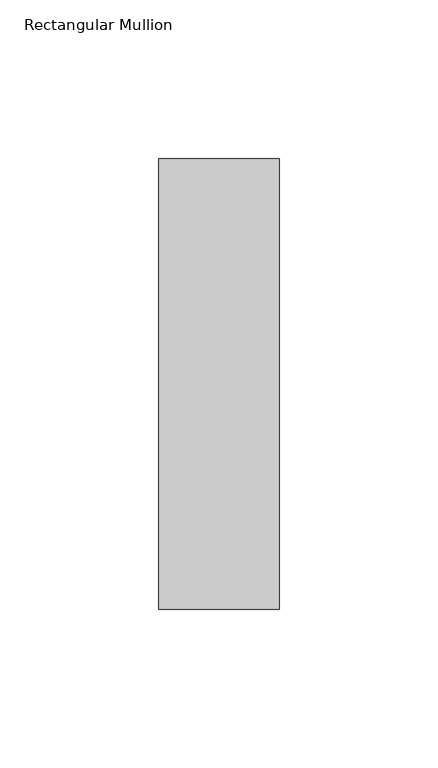
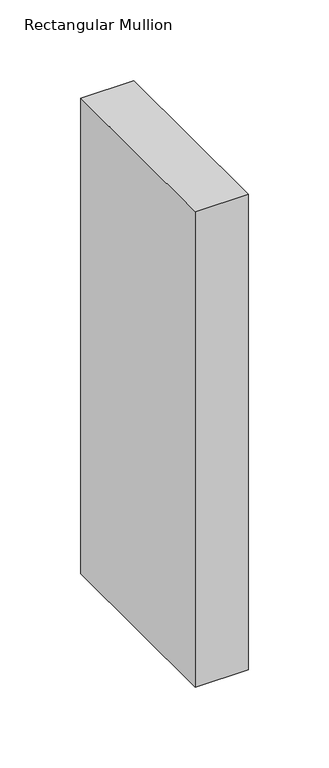
"""IFC4 building model written with IfcOpenShell, lengths in millimetres: member geometry, Rectangular Mullion : NLRS_21_CWM_hsb-regel 38x142_gen_rsf."""

from ifc_helpers import new_model, si_unit, frame, origin, place, context, project, spatial, polyline, outline, extrude, source, transform, mapped, element, save


def rectangular_mullion_923ec213(model_context):
    return source(origin(), model_context, "Body", "SweptSolid", [
        extrude(outline(polyline([(0.0, -71.0), (-38.0, -71.0), (-38.0, 71.0), (0.0, 71.0), (0.0, -71.0)])), frame((0.0, 0.0, -359.9999997), z_axis=(0.0, 0.0, 1.0), x_axis=(1.0, 0.0, 0.0)), (0.0, 0.0, 1.0), 359.9999997),
    ])


if __name__ == "__main__":
    model = new_model("IFC4")
    model_context = context("Model", 3, world=origin())
    ifc_project = project(units=[si_unit("LENGTHUNIT", "METRE", prefix="MILLI")], contexts=[model_context])
    site = spatial("IfcSite", under=ifc_project)
    building = spatial("IfcBuilding", under=site)
    placement = place(None, origin())
    rectangular_mullion_shape = rectangular_mullion_923ec213(model_context)
    element("IfcMember", 1, ObjectType="Rectangular Mullion : NLRS_21_CWM_hsb-regel 38x142_gen_rsf", at=placement, inside=building, context=model_context, shape_type="MappedRepresentation", body=[
        mapped(rectangular_mullion_shape, transform((0.0, 0.0, 0.0), x_axis=(1.0, 0.0, 0.0), y_axis=(0.0, 1.0, 0.0), z_axis=(0.0, 0.0, 1.0))),
    ])
    save(model, "model.ifc")

# Revit data of these elements
# Type "Rectangular Mullion : NLRS_21_CWM_hsb-regel 38x142_gen_rsf"
#   Export Type to IFC As = "IfcWall"
#   Type IfcGUID = "07M7mRoiH1CR8m_RSKIwpF"
#   Assembly Code = "21.10"
#   built-in parameter 1007322 = 0.465879 (stored number, unit not read)
#   built-in parameter 1007321 = 0.062336 (stored number, unit not read)
#   built-in parameter 1007320 = 0.062336 (stored number, unit not read)
# Element 1 (IfcMember, "Rectangular Mullion : NLRS_21_CWM_hsb-regel 38x142_gen_rsf")
#   Materials on its faces: "NLRS_i2_hout naaldhout vuren_gen_rsf"
# Materials
#   "NLRS_i2_hout naaldhout vuren_gen_rsf": class "I - Hout", colour RGB 234 199 147, transparency 0, Keynote = "i2", Manufacturer = "Revit Standards Foundation", URL = "www.revitstandards.org", Description = "hout vuren", Cost = 0
